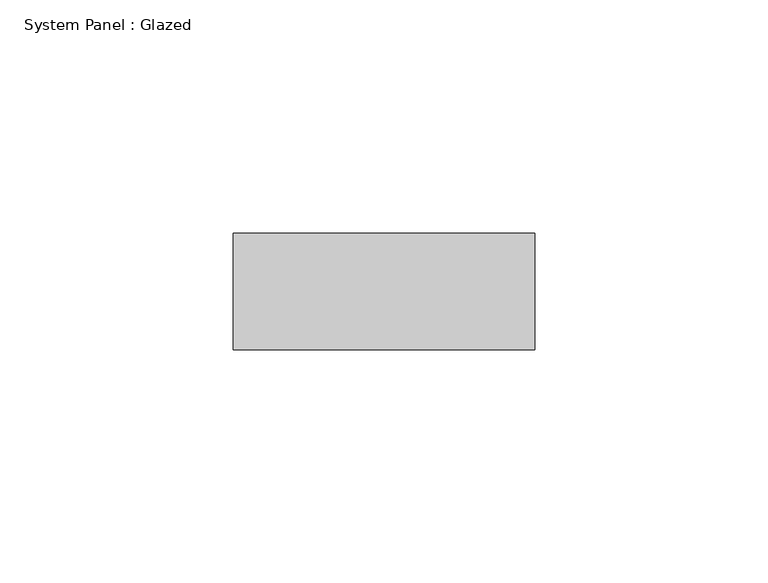
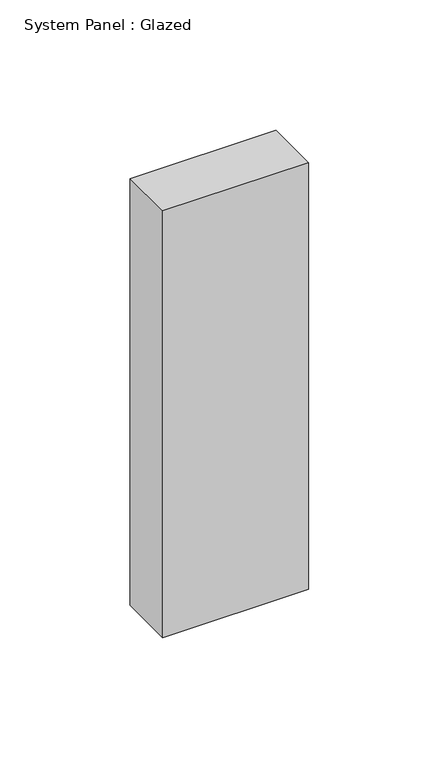
"""IFC4 building model written with IfcOpenShell, lengths in millimetres: plate geometry, System Panel : Glazed."""

from ifc_helpers import new_model, si_unit, origin, origin_with_axes, place, context, project, spatial, polyline, outline, extrude, source, transform, mapped, element, save


def system_panel_glazed_d23853e5(model_context):
    return source(origin(), model_context, "Body", "SweptSolid", [
        extrude(outline(polyline([(32.3630881, 24.5), (-32.3630881, 24.5), (-32.3630881, 49.5), (32.3630881, 49.5), (32.3630881, 24.5)])), origin_with_axes(), (0.0, 0.0, 1.0), 200.0),
    ])


if __name__ == "__main__":
    model = new_model("IFC4")
    model_context = context("Model", 3, world=origin())
    ifc_project = project(units=[si_unit("LENGTHUNIT", "METRE", prefix="MILLI")], contexts=[model_context])
    site = spatial("IfcSite", under=ifc_project)
    building = spatial("IfcBuilding", under=site)
    placement = place(None, origin())
    system_panel_glazed_shape = system_panel_glazed_d23853e5(model_context)
    element("IfcPlate", 1, ObjectType="System Panel : Glazed", at=placement, inside=building, context=model_context, shape_type="MappedRepresentation", body=[
        mapped(system_panel_glazed_shape, transform((0.0, 0.0, 0.0), x_axis=(1.0, 0.0, 0.0), y_axis=(0.0, 1.0, 0.0), z_axis=(0.0, 0.0, 1.0))),
    ])
    save(model, "model.ifc")

# Revit data of these elements
# Element 1 (IfcPlate, "System Panel : Glazed")
#   Materials on its faces: "Glass"
# Materials
#   "Glass": class "Glass", colour RGB 218 227 224, transparency 0.85, Description = "Soda Lime Glass", Cost = 0
